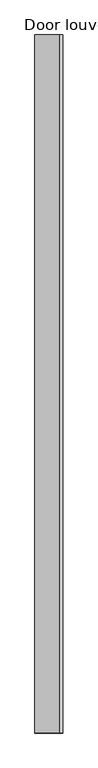
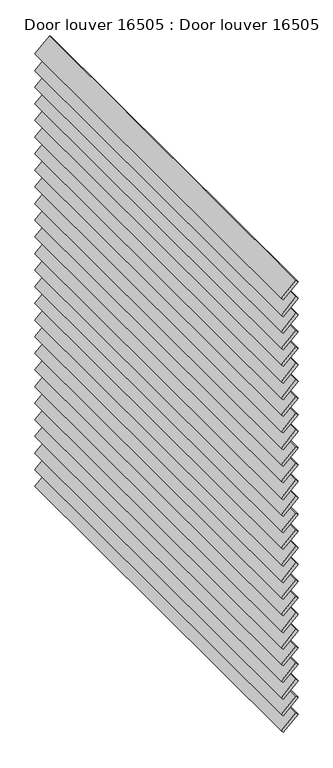
"""IFC4 building model written with IfcOpenShell, lengths in millimetres: proxy geometry, Door louver 16505 : Door louver 16505."""

import ifcopenshell
import ifcopenshell.guid

model = None  # the IFC model being written
_history = None  # IfcOwnerHistory: only IFC2X3 demands one
_inside = {}  # id of a spatial element -> (the spatial element, [elements in it])
_under = {}  # id of a project, library or spatial element -> (it, [spatial elements below it])
_declared = {}  # id of a project -> (the project, [libraries it declares])
_typed = {}  # id of a type object -> (the type object, [elements of that type])
_made_of = {}  # id of a material, layer set ... -> (it, [elements and type objects made of it])


def new_model(schema):
    """Start an empty IFC model of exactly this schema.

    Asked for "IFC4X3", IfcOpenShell would pick the latest addendum, in which some entities
    have other attributes; the version numbers below select the first issue.
    IFC2X3 requires an IfcOwnerHistory on every rooted entity: one is made here for all.
    """
    global model, _history
    if schema == "IFC4X3":
        model = ifcopenshell.file(schema_version=(4, 3, 0, 0))
    else:
        model = ifcopenshell.file(schema=schema)
    _inside.clear()
    _under.clear()
    _declared.clear()
    _typed.clear()
    _made_of.clear()
    _history = None
    if model.schema == "IFC2X3":
        org = make("IfcOrganization", Name="unknown")
        user = make(
            "IfcPersonAndOrganization",
            ThePerson=make("IfcPerson", FamilyName="unknown"),
            TheOrganization=org,
        )
        app = make(
            "IfcApplication",
            ApplicationDeveloper=org,
            Version="unknown",
            ApplicationFullName="unknown",
            ApplicationIdentifier="unknown",
        )
        _history = make(
            "IfcOwnerHistory",
            OwningUser=user,
            OwningApplication=app,
            ChangeAction="ADDED",
            CreationDate=0,
        )
    return model


def make(cls, **values):
    """One entity of the class cls with the attributes given. An attribute that is None is left unset."""
    return model.create_entity(
        cls, **{name: value for name, value in values.items() if value is not None}
    )


def rooted(cls, **values):
    """An entity with a GlobalId (a new one), such as an element, a storey or a relation."""
    return make(cls, GlobalId=ifcopenshell.guid.new(), OwnerHistory=_history, **values)


def si_unit(unit_type, name, prefix=None):
    """IfcSIUnit, for example si_unit("LENGTHUNIT", "METRE", prefix="MILLI")."""
    return make("IfcSIUnit", UnitType=unit_type, Prefix=prefix, Name=name)


def assignment(units):
    """IfcUnitAssignment: the units of a project."""
    return None if units is None else make("IfcUnitAssignment", Units=units)


def point(xyz):
    """IfcCartesianPoint."""
    return None if xyz is None else make("IfcCartesianPoint", Coordinates=xyz)


def direction(xyz):
    """IfcDirection."""
    return None if xyz is None else make("IfcDirection", DirectionRatios=xyz)


def frame(location, z_axis=None, x_axis=None):
    """IfcAxis2Placement3D, a coordinate frame: its origin and axes. An axis left out is left unset."""
    return make(
        "IfcAxis2Placement3D",
        Location=point(location),
        Axis=direction(z_axis),
        RefDirection=direction(x_axis),
    )


def origin():
    """The frame at (0, 0, 0) with its axes left unset."""
    return frame((0.0, 0.0, 0.0))


def place(relative_to, where):
    """IfcLocalPlacement: puts the frame where relative to a parent placement (None: the world)."""
    return make(
        "IfcLocalPlacement", PlacementRelTo=relative_to, RelativePlacement=where
    )


def context(
    kind, dimensions, precision=None, world=None, true_north=None, identifier=None
):
    """IfcGeometricRepresentationContext, for example the 3D "Model" context."""
    return make(
        "IfcGeometricRepresentationContext",
        ContextIdentifier=identifier,
        ContextType=kind,
        CoordinateSpaceDimension=dimensions,
        Precision=precision,
        WorldCoordinateSystem=world,
        TrueNorth=true_north,
    )


def project(units=None, contexts=None):
    """IfcProject with its units and contexts."""
    return rooted(
        "IfcProject",
        Name="project",
        RepresentationContexts=contexts,
        UnitsInContext=assignment(units),
    )


def spatial(cls, under=None, at=None, **own):
    """A site, building, storey or space (cls), placed at a placement, below another one or the project."""
    s = rooted(cls, ObjectPlacement=at, **own)
    if under is not None:
        _under.setdefault(under.id(), (under, []))[1].append(s)
    return s


def polyline(points):
    """IfcPolyline through the points."""
    return make("IfcPolyline", Points=[point(p) for p in points])


def outline(outer, holes=None, kind="AREA"):
    """IfcArbitraryClosedProfileDef: a profile drawn as a closed curve; with holes, ...WithVoids."""
    if holes is None:
        return make("IfcArbitraryClosedProfileDef", ProfileType=kind, OuterCurve=outer)
    return make(
        "IfcArbitraryProfileDefWithVoids",
        ProfileType=kind,
        OuterCurve=outer,
        InnerCurves=holes,
    )


def extrude(swept, where, along, depth):
    """IfcExtrudedAreaSolid: the profile swept, set in the frame where, extruded along a direction by depth."""
    return make(
        "IfcExtrudedAreaSolid",
        SweptArea=swept,
        Position=where,
        ExtrudedDirection=direction(along),
        Depth=depth,
    )


def shape(context_of_items, identifier, shape_type, items):
    """IfcShapeRepresentation: the items that make up one representation, for example the "Body"."""
    return make(
        "IfcShapeRepresentation",
        ContextOfItems=context_of_items,
        RepresentationIdentifier=identifier,
        RepresentationType=shape_type,
        Items=items,
    )


def source(mapping_origin, context_of_items, identifier, shape_type, items):
    """IfcRepresentationMap: a shape defined once, which mapped items show again and again."""
    return make(
        "IfcRepresentationMap",
        MappingOrigin=mapping_origin,
        MappedRepresentation=shape(context_of_items, identifier, shape_type, items),
    )


def transform(
    local_origin,
    x_axis=None,
    y_axis=None,
    z_axis=None,
    scale=None,
    scale2=None,
    scale3=None,
    uniform=True,
):
    """IfcCartesianTransformationOperator3D, or its non-uniform kind. x_axis, y_axis, z_axis: its Axis1, 2, 3."""
    if uniform:
        return make(
            "IfcCartesianTransformationOperator3D",
            Axis1=direction(x_axis),
            Axis2=direction(y_axis),
            LocalOrigin=point(local_origin),
            Scale=scale,
            Axis3=direction(z_axis),
        )
    return make(
        "IfcCartesianTransformationOperator3DnonUniform",
        Axis1=direction(x_axis),
        Axis2=direction(y_axis),
        LocalOrigin=point(local_origin),
        Scale=scale,
        Axis3=direction(z_axis),
        Scale2=scale2,
        Scale3=scale3,
    )


def mapped(mapping_source, mapping_target):
    """IfcMappedItem: shows the shape of a source again, moved by a transform."""
    return make(
        "IfcMappedItem", MappingSource=mapping_source, MappingTarget=mapping_target
    )


def made_of(thing, what):
    """Note that an element or type object is made of a material, layer set ...; save() writes the relation."""
    if what is not None:
        _made_of.setdefault(what.id(), (what, []))[1].append(thing)
    return thing


def element(
    cls,
    number,
    at=None,
    inside=None,
    cuts=None,
    type_object=None,
    material=None,
    context=None,
    identifier="Body",
    shape_type=None,
    held_by="IfcProductDefinitionShape",
    body=None,
    shapes=None,
    **own,
):
    """One element of the class cls, such as IfcWall. Its Tag is "e" and its number.

    at: its placement. inside: the storey or other place that contains it. cuts: it is an
    opening in that element (IfcRelVoidsElement). A single representation is given by context,
    identifier, shape_type and body (its items); several are given by shapes. held_by: the class
    of the entity that holds the representations. save() writes the other relations.
    """
    e = rooted(cls, Tag="e%d" % number, ObjectPlacement=at, **own)
    if body is not None:
        shapes = [shape(context, identifier, shape_type, body)]
    if shapes is not None:
        e.Representation = make(held_by, Representations=shapes)
    if inside is not None:
        _inside.setdefault(inside.id(), (inside, []))[1].append(e)
    if cuts is not None:
        rooted(
            "IfcRelVoidsElement", RelatingBuildingElement=cuts, RelatedOpeningElement=e
        )
    if type_object is not None:
        _typed.setdefault(type_object.id(), (type_object, []))[1].append(e)
    return made_of(e, material)


def aggregate(whole, parts):
    """IfcRelAggregates: a whole, such as a stair, and the parts it consists of."""
    return rooted("IfcRelAggregates", RelatingObject=whole, RelatedObjects=parts)


def save(model, path):
    """Write the relations noted so far, then the file.

    IfcRelAggregates (storeys below a building ...), IfcRelContainedInSpatialStructure (elements
    in a storey), IfcRelDefinesByType, IfcRelAssociatesMaterial and IfcRelDeclares: one each for
    every whole, place, type object, material and project.
    """
    for whole, parts in _under.values():
        aggregate(whole, parts)
    for where, things in _inside.values():
        rooted(
            "IfcRelContainedInSpatialStructure",
            RelatedElements=things,
            RelatingStructure=where,
        )
    for kind, things in _typed.values():
        rooted("IfcRelDefinesByType", RelatedObjects=things, RelatingType=kind)
    for what, things in _made_of.values():
        rooted("IfcRelAssociatesMaterial", RelatedObjects=things, RelatingMaterial=what)
    for by, libraries in _declared.values():
        rooted("IfcRelDeclares", RelatingContext=by, RelatedDefinitions=libraries)
    model.write(path)


def door_louver_16505_door_louver_16505_d946a3b7(model_context):
    return source(origin(), model_context, "Body", "SweptSolid", [
        extrude(outline(polyline([(0.0, -88.6), (0.0, 0.0), (1847.6, 0.0), (1847.6, -88.6), (0.0, -88.6)])), frame((-8304.3306423, 6540.4513244, 32854.8547367), z_axis=(-0.6925092278135618, 0.0, 0.721409016711785), x_axis=(0.0, -1.0, 0.0)), (0.0, 0.0, 1.0), 13.8216714),
        extrude(outline(polyline([(0.0, -88.6), (0.0, 0.0), (1847.6, 0.0), (1847.6, -88.6), (0.0, -88.6)])), frame((-8304.3306423, 6540.4513244, 32931.0547367), z_axis=(-0.6925092278135618, 0.0, 0.721409016711785), x_axis=(0.0, -1.0, 0.0)), (0.0, 0.0, 1.0), 13.8216714),
        extrude(outline(polyline([(0.0, -88.6), (0.0, 0.0), (1847.6, 0.0), (1847.6, -88.6), (0.0, -88.6)])), frame((-8304.3306423, 6540.4513244, 33007.2547367), z_axis=(-0.6925092278135618, 0.0, 0.721409016711785), x_axis=(0.0, -1.0, 0.0)), (0.0, 0.0, 1.0), 13.8216714),
        extrude(outline(polyline([(0.0, -88.6), (0.0, 0.0), (1847.6, 0.0), (1847.6, -88.6), (0.0, -88.6)])), frame((-8304.3306423, 6540.4513244, 33083.4547367), z_axis=(-0.6925092278135618, 0.0, 0.721409016711785), x_axis=(0.0, -1.0, 0.0)), (0.0, 0.0, 1.0), 13.8216714),
        extrude(outline(polyline([(0.0, -88.6), (0.0, 0.0), (1847.6, 0.0), (1847.6, -88.6), (0.0, -88.6)])), frame((-8304.3306423, 6540.4513244, 33159.6547367), z_axis=(-0.6925092278135618, 0.0, 0.721409016711785), x_axis=(0.0, -1.0, 0.0)), (0.0, 0.0, 1.0), 13.8216714),
        extrude(outline(polyline([(0.0, -88.6), (0.0, 0.0), (1847.6, 0.0), (1847.6, -88.6), (0.0, -88.6)])), frame((-8304.3306423, 6540.4513244, 33235.8547367), z_axis=(-0.6925092278135618, 0.0, 0.721409016711785), x_axis=(0.0, -1.0, 0.0)), (0.0, 0.0, 1.0), 13.8216714),
        extrude(outline(polyline([(0.0, -88.6), (0.0, 0.0), (1847.6, 0.0), (1847.6, -88.6), (0.0, -88.6)])), frame((-8304.3306423, 6540.4513244, 33312.0547367), z_axis=(-0.6925092278135618, 0.0, 0.721409016711785), x_axis=(0.0, -1.0, 0.0)), (0.0, 0.0, 1.0), 13.8216714),
        extrude(outline(polyline([(0.0, -88.6), (0.0, 0.0), (1847.6, 0.0), (1847.6, -88.6), (0.0, -88.6)])), frame((-8304.3306423, 6540.4513244, 33388.2547367), z_axis=(-0.6925092278135618, 0.0, 0.721409016711785), x_axis=(0.0, -1.0, 0.0)), (0.0, 0.0, 1.0), 13.8216714),
        extrude(outline(polyline([(0.0, -88.6), (0.0, 0.0), (1847.6, 0.0), (1847.6, -88.6), (0.0, -88.6)])), frame((-8304.3306423, 6540.4513244, 33464.4547367), z_axis=(-0.6925092278135618, 0.0, 0.721409016711785), x_axis=(0.0, -1.0, 0.0)), (0.0, 0.0, 1.0), 13.8216714),
        extrude(outline(polyline([(0.0, -88.6), (0.0, 0.0), (1847.6, 0.0), (1847.6, -88.6), (0.0, -88.6)])), frame((-8304.3306423, 6540.4513244, 33540.6547367), z_axis=(-0.6925092278135618, 0.0, 0.721409016711785), x_axis=(0.0, -1.0, 0.0)), (0.0, 0.0, 1.0), 13.8216714),
        extrude(outline(polyline([(0.0, -88.6), (0.0, 0.0), (1847.6, 0.0), (1847.6, -88.6), (0.0, -88.6)])), frame((-8304.3306423, 6540.4513244, 33616.8547367), z_axis=(-0.6925092278135618, 0.0, 0.721409016711785), x_axis=(0.0, -1.0, 0.0)), (0.0, 0.0, 1.0), 13.8216714),
        extrude(outline(polyline([(0.0, -88.6), (0.0, 0.0), (1847.6, 0.0), (1847.6, -88.6), (0.0, -88.6)])), frame((-8304.3306423, 6540.4513244, 33693.0547367), z_axis=(-0.6925092278135618, 0.0, 0.721409016711785), x_axis=(0.0, -1.0, 0.0)), (0.0, 0.0, 1.0), 13.8216714),
        extrude(outline(polyline([(0.0, -88.6), (0.0, 0.0), (1847.6, 0.0), (1847.6, -88.6), (0.0, -88.6)])), frame((-8304.3306423, 6540.4513244, 33769.2547367), z_axis=(-0.6925092278135618, 0.0, 0.721409016711785), x_axis=(0.0, -1.0, 0.0)), (0.0, 0.0, 1.0), 13.8216714),
        extrude(outline(polyline([(0.0, -88.6), (0.0, 0.0), (1847.6, 0.0), (1847.6, -88.6), (0.0, -88.6)])), frame((-8304.3306423, 6540.4513244, 33845.4547367), z_axis=(-0.6925092278135618, 0.0, 0.721409016711785), x_axis=(0.0, -1.0, 0.0)), (0.0, 0.0, 1.0), 13.8216714),
        extrude(outline(polyline([(0.0, -88.6), (0.0, 0.0), (1847.6, 0.0), (1847.6, -88.6), (0.0, -88.6)])), frame((-8304.3306423, 6540.4513244, 33921.6547367), z_axis=(-0.6925092278135618, 0.0, 0.721409016711785), x_axis=(0.0, -1.0, 0.0)), (0.0, 0.0, 1.0), 13.8216714),
        extrude(outline(polyline([(0.0, -88.6), (0.0, 0.0), (1847.6, 0.0), (1847.6, -88.6), (0.0, -88.6)])), frame((-8304.3306423, 6540.4513244, 33997.8547367), z_axis=(-0.6925092278135618, 0.0, 0.721409016711785), x_axis=(0.0, -1.0, 0.0)), (0.0, 0.0, 1.0), 13.8216714),
        extrude(outline(polyline([(0.0, -88.6), (0.0, 0.0), (1847.6, 0.0), (1847.6, -88.6), (0.0, -88.6)])), frame((-8304.3306423, 6540.4513244, 34074.0547367), z_axis=(-0.6925092278135618, 0.0, 0.721409016711785), x_axis=(0.0, -1.0, 0.0)), (0.0, 0.0, 1.0), 13.8216714),
        extrude(outline(polyline([(0.0, -88.6), (0.0, 0.0), (1847.6, 0.0), (1847.6, -88.6), (0.0, -88.6)])), frame((-8304.3306423, 6540.4513244, 34150.2547367), z_axis=(-0.6925092278135618, 0.0, 0.721409016711785), x_axis=(0.0, -1.0, 0.0)), (0.0, 0.0, 1.0), 13.8216714),
        extrude(outline(polyline([(0.0, -88.6), (0.0, 0.0), (1847.6, 0.0), (1847.6, -88.6), (0.0, -88.6)])), frame((-8304.3306423, 6540.4513244, 34226.4547367), z_axis=(-0.6925092278135618, 0.0, 0.721409016711785), x_axis=(0.0, -1.0, 0.0)), (0.0, 0.0, 1.0), 13.8216714),
        extrude(outline(polyline([(0.0, -88.6), (0.0, 0.0), (1847.6, 0.0), (1847.6, -88.6), (0.0, -88.6)])), frame((-8304.3306423, 6540.4513244, 34302.6547367), z_axis=(-0.6925092278135618, 0.0, 0.721409016711785), x_axis=(0.0, -1.0, 0.0)), (0.0, 0.0, 1.0), 13.8216714),
        extrude(outline(polyline([(0.0, -88.6), (0.0, 0.0), (1847.6, 0.0), (1847.6, -88.6), (0.0, -88.6)])), frame((-8304.3306423, 6540.4513244, 34378.8547367), z_axis=(-0.6925092278135618, 0.0, 0.721409016711785), x_axis=(0.0, -1.0, 0.0)), (0.0, 0.0, 1.0), 13.8216714),
        extrude(outline(polyline([(0.0, -88.6), (0.0, 0.0), (1847.6, 0.0), (1847.6, -88.6), (0.0, -88.6)])), frame((-8304.3306423, 6540.4513244, 34455.0547367), z_axis=(-0.6925092278135618, 0.0, 0.721409016711785), x_axis=(0.0, -1.0, 0.0)), (0.0, 0.0, 1.0), 13.8216714),
        extrude(outline(polyline([(0.0, -88.6), (0.0, 0.0), (1847.6, 0.0), (1847.6, -88.6), (0.0, -88.6)])), frame((-8304.3306423, 6540.4513244, 34531.2547367), z_axis=(-0.6925092278135618, 0.0, 0.721409016711785), x_axis=(0.0, -1.0, 0.0)), (0.0, 0.0, 1.0), 13.8216714),
        extrude(outline(polyline([(0.0, -88.6), (0.0, 0.0), (1847.6, 0.0), (1847.6, -88.6), (0.0, -88.6)])), frame((-8304.3306423, 6540.4513244, 34607.4547367), z_axis=(-0.6925092278135618, 0.0, 0.721409016711785), x_axis=(0.0, -1.0, 0.0)), (0.0, 0.0, 1.0), 13.8216714),
        extrude(outline(polyline([(0.0, -88.6), (0.0, 0.0), (1847.6, 0.0), (1847.6, -88.6), (0.0, -88.6)])), frame((-8304.3306423, 6540.4513244, 34683.6547367), z_axis=(-0.6925092278135618, 0.0, 0.721409016711785), x_axis=(0.0, -1.0, 0.0)), (0.0, 0.0, 1.0), 13.8216714),
        extrude(outline(polyline([(0.0, -88.6), (0.0, 0.0), (1847.6, 0.0), (1847.6, -88.6), (0.0, -88.6)])), frame((-8304.3306423, 6540.4513244, 34759.8547367), z_axis=(-0.6925092278135618, 0.0, 0.721409016711785), x_axis=(0.0, -1.0, 0.0)), (0.0, 0.0, 1.0), 13.8216714),
        extrude(outline(polyline([(0.0, -88.6), (0.0, 0.0), (1847.6, 0.0), (1847.6, -88.6), (0.0, -88.6)])), frame((-8304.3306423, 6540.4513244, 34836.0547367), z_axis=(-0.6925092278135618, 0.0, 0.721409016711785), x_axis=(0.0, -1.0, 0.0)), (0.0, 0.0, 1.0), 13.8216714),
    ])


if __name__ == "__main__":
    model = new_model("IFC4")
    model_context = context("Model", 3, world=origin())
    ifc_project = project(units=[si_unit("LENGTHUNIT", "METRE", prefix="MILLI")], contexts=[model_context])
    site = spatial("IfcSite", under=ifc_project)
    building = spatial("IfcBuilding", under=site)
    placement = place(None, origin())
    door_louver_16505_door_louver_16505_shape = door_louver_16505_door_louver_16505_d946a3b7(model_context)
    element("IfcBuildingElementProxy", 1, Name="Door louver 16505 : Door louver 16505", ObjectType="Door louver 16505 : Door louver 16505", at=placement, inside=building, context=model_context, shape_type="MappedRepresentation", body=[
        mapped(door_louver_16505_door_louver_16505_shape, transform((0.0, 0.0, 0.0), x_axis=(1.0, 0.0, 0.0), y_axis=(0.0, 1.0, 0.0), z_axis=(0.0, 0.0, 1.0))),
    ])
    save(model, "model.ifc")

# Revit data of these elements
# Type "Door louver 16505 : Door louver 16505"
#   NameOverride = "Door louver"
# Element 1 (IfcBuildingElementProxy, "Door louver 16505 : Door louver 16505")
#   Materials on its faces: "WOODEN LOUVERS (SPEC T. B. D.)"
# Materials
#   "WOODEN LOUVERS (SPEC T. B. D.)": class "Unassigned", colour RGB 148 103 60, transparency 0, Cost = 0
